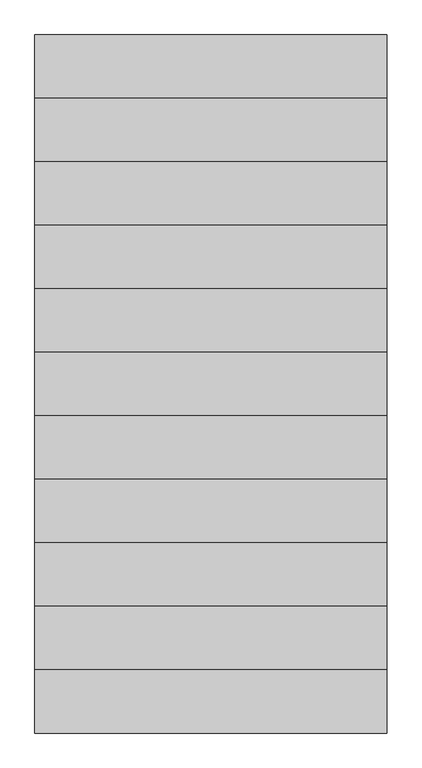
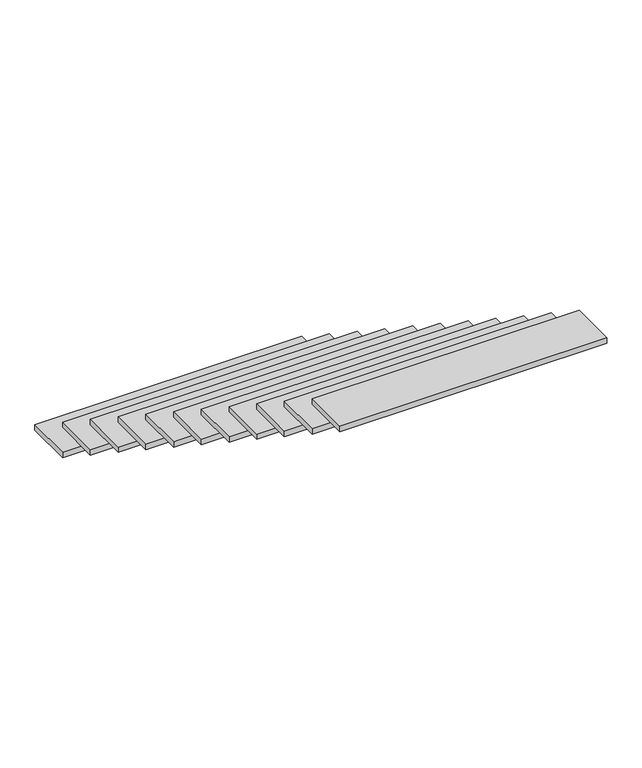
"""IFC4 building model written with IfcOpenShell, lengths in millimetres: stair flight geometry."""

from ifc_helpers import new_model, si_unit, frame, origin, place, context, project, spatial, polyline, outline, extrude, source, transform, mapped, element, save


def stair_flight_7c2b7268(model_context):
    return source(origin(), model_context, "Body", "SweptSolid", [
        extrude(outline(polyline([(16085.3403387, 4647.6066446), (14585.3403387, 4647.6066446), (14585.3403387, 4917.6066446), (16085.3403387, 4917.6066446), (16085.3403387, 4647.6066446)])), frame((0.0, 0.0, 13939.4285714), z_axis=(0.0, 0.0, 1.0), x_axis=(1.0, 0.0, 0.0)), (0.0, 0.0, 1.0), 32.0),
        extrude(outline(polyline([(16085.3403387, 4377.6066446), (14585.3403387, 4377.6066446), (14585.3403387, 4647.6066446), (16085.3403387, 4647.6066446), (16085.3403387, 4377.6066446)])), frame((0.0, 0.0, 14118.5494505), z_axis=(0.0, 0.0, 1.0), x_axis=(1.0, 0.0, 0.0)), (0.0, 0.0, 1.0), 32.0),
        extrude(outline(polyline([(16085.3403387, 4107.6066446), (14585.3403387, 4107.6066446), (14585.3403387, 4377.6066446), (16085.3403387, 4377.6066446), (16085.3403387, 4107.6066446)])), frame((0.0, 0.0, 14297.6703297), z_axis=(0.0, 0.0, 1.0), x_axis=(1.0, 0.0, 0.0)), (0.0, 0.0, 1.0), 32.0),
        extrude(outline(polyline([(16085.3403387, 3837.6066446), (14585.3403387, 3837.6066446), (14585.3403387, 4107.6066446), (16085.3403387, 4107.6066446), (16085.3403387, 3837.6066446)])), frame((0.0, 0.0, 14476.7912088), z_axis=(0.0, 0.0, 1.0), x_axis=(1.0, 0.0, 0.0)), (0.0, 0.0, 1.0), 32.0),
        extrude(outline(polyline([(16085.3403387, 3567.6066446), (14585.3403387, 3567.6066446), (14585.3403387, 3837.6066446), (16085.3403387, 3837.6066446), (16085.3403387, 3567.6066446)])), frame((0.0, 0.0, 14655.9120879), z_axis=(0.0, 0.0, 1.0), x_axis=(1.0, 0.0, 0.0)), (0.0, 0.0, 1.0), 32.0),
        extrude(outline(polyline([(16085.3403387, 3297.6066446), (14585.3403387, 3297.6066446), (14585.3403387, 3567.6066446), (16085.3403387, 3567.6066446), (16085.3403387, 3297.6066446)])), frame((0.0, 0.0, 14835.032967), z_axis=(0.0, 0.0, 1.0), x_axis=(1.0, 0.0, 0.0)), (0.0, 0.0, 1.0), 32.0),
        extrude(outline(polyline([(16085.3403387, 3027.6066446), (14585.3403387, 3027.6066446), (14585.3403387, 3297.6066446), (16085.3403387, 3297.6066446), (16085.3403387, 3027.6066446)])), frame((0.0, 0.0, 15014.1538462), z_axis=(0.0, 0.0, 1.0), x_axis=(1.0, 0.0, 0.0)), (0.0, 0.0, 1.0), 32.0),
        extrude(outline(polyline([(16085.3403387, 2757.6066446), (14585.3403387, 2757.6066446), (14585.3403387, 3027.6066446), (16085.3403387, 3027.6066446), (16085.3403387, 2757.6066446)])), frame((0.0, 0.0, 15193.2747253), z_axis=(0.0, 0.0, 1.0), x_axis=(1.0, 0.0, 0.0)), (0.0, 0.0, 1.0), 32.0),
        extrude(outline(polyline([(16085.3403387, 2487.6066446), (14585.3403387, 2487.6066446), (14585.3403387, 2757.6066446), (16085.3403387, 2757.6066446), (16085.3403387, 2487.6066446)])), frame((0.0, 0.0, 15372.3956044), z_axis=(0.0, 0.0, 1.0), x_axis=(1.0, 0.0, 0.0)), (0.0, 0.0, 1.0), 32.0),
        extrude(outline(polyline([(16085.3403387, 2217.6066446), (14585.3403387, 2217.6066446), (14585.3403387, 2487.6066446), (16085.3403387, 2487.6066446), (16085.3403387, 2217.6066446)])), frame((0.0, 0.0, 15551.5164835), z_axis=(0.0, 0.0, 1.0), x_axis=(1.0, 0.0, 0.0)), (0.0, 0.0, 1.0), 32.0),
        extrude(outline(polyline([(16085.3403387, 1947.6066446), (14585.3403387, 1947.6066446), (14585.3403387, 2217.6066446), (16085.3403387, 2217.6066446), (16085.3403387, 1947.6066446)])), frame((0.0, 0.0, 15730.6373626), z_axis=(0.0, 0.0, 1.0), x_axis=(1.0, 0.0, 0.0)), (0.0, 0.0, 1.0), 32.0),
    ])


if __name__ == "__main__":
    model = new_model("IFC4")
    model_context = context("Model", 3, world=origin())
    ifc_project = project(units=[si_unit("LENGTHUNIT", "METRE", prefix="MILLI")], contexts=[model_context])
    site = spatial("IfcSite", under=ifc_project)
    building = spatial("IfcBuilding", under=site)
    placement = place(None, origin())
    stair_flight_shape = stair_flight_7c2b7268(model_context)
    element("IfcStairFlight", 1, at=placement, inside=building, context=model_context, shape_type="MappedRepresentation", body=[
        mapped(stair_flight_shape, transform((0.0, 0.0, 0.0), x_axis=(1.0, 0.0, 0.0), y_axis=(0.0, 1.0, 0.0), z_axis=(0.0, 0.0, 1.0))),
    ])
    save(model, "model.ifc")

# Revit data of these elements
# Element 1 (IfcStairFlight)
#   Materials on its faces: "철강"
# Materials
#   "철강": class "Generic", colour RGB 143 142 141, transparency 0, Description = "철골+가공조립+세우기", Cost = 0
